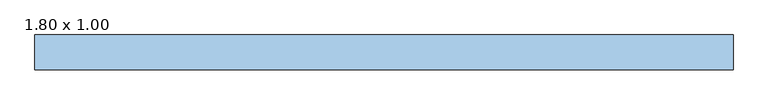
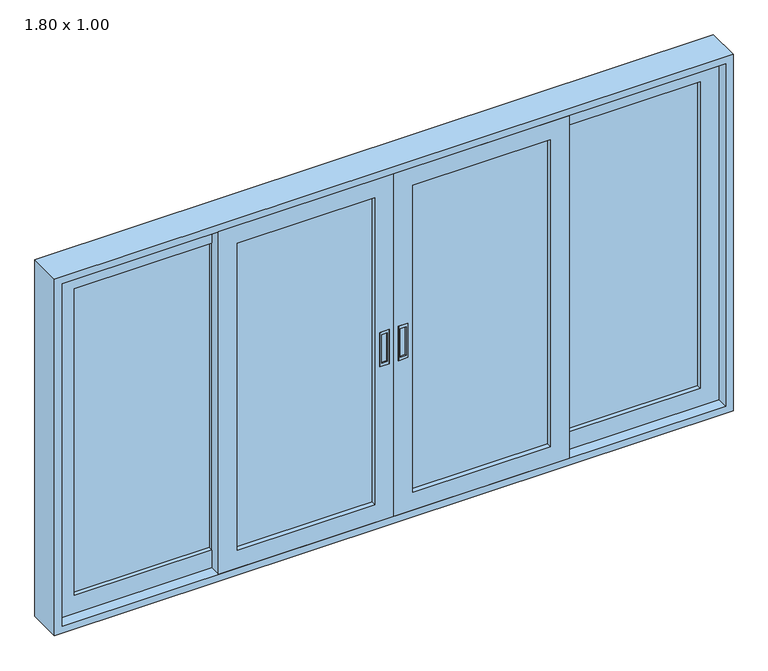
"""IFC4 building model written with IfcOpenShell, lengths in millimetres: window geometry, CC_JANELA CORRER_4 FOLHAS VIDRO : 1.80 x 1.00."""

from ifc_helpers import new_model, si_unit, frame, origin, place, context, project, spatial, polyline, outline, extrude, faceted_brep, source, transform, mapped, element, save


def window_1_80_x_1_00_ac21060c(model_context):
    return source(origin(), model_context, "Body", "SolidModel", [
        extrude(outline(polyline([(17.5, -96.0), (17.5, -95.0), (32.5, -95.0), (32.5, -96.0), (17.5, -96.0)])), frame((0.0, 0.0, 1460.0), z_axis=(0.0, 0.0, 1.0), x_axis=(1.0, 0.0, 0.0)), (0.0, 0.0, 1.0), 80.0),
        extrude(outline(polyline([(1452.0, 37.5), (1548.0, 37.5), (1548.0, 12.5), (1452.0, 12.5), (1452.0, 37.5)]), holes=[polyline([(1460.0, 32.5), (1460.0, 17.5), (1540.0, 17.5), (1540.0, 32.5), (1460.0, 32.5)])]), frame((0.0, -100.1, 0.0), z_axis=(0.0, 1.0, 0.0), x_axis=(0.0, 0.0, 1.0)), (0.0, 0.0, 1.0), 5.1),
        faceted_brep([(50.0, -100.0, 1930.0), (50.0, -100.0, 1070.0), (50.0, -70.0, 1070.0), (50.0, -70.0, 1930.0), (0.0, -70.0, 1980.0), (465.0, -70.0, 1980.0), (465.0, -70.0, 1020.0), (0.0, -70.0, 1020.0), (415.0, -70.0, 1070.0), (415.0, -70.0, 1930.0), (415.0, -100.0, 1070.0), (0.0, -100.0, 1020.0), (465.0, -100.0, 1020.0), (465.0, -100.0, 1980.0), (0.0, -100.0, 1980.0), (37.5, -100.0, 1548.0), (37.5, -100.0, 1452.0), (12.5, -100.0, 1452.0), (12.5, -100.0, 1548.0), (415.0, -100.0, 1930.0), (12.5, -95.0, 1452.0), (12.5, -95.0, 1548.0), (37.5, -95.0, 1452.0), (37.5, -95.0, 1548.0)], [[[0, 1, 2, 3]], [[4, 5, 6, 7], [2, 8, 9, 3]], [[1, 10, 8, 2]], [[11, 12, 13, 14], [15, 16, 17, 18], [0, 19, 10, 1]], [[4, 7, 11, 14]], [[7, 6, 12, 11]], [[10, 19, 9, 8]], [[6, 5, 13, 12]], [[18, 17, 20, 21]], [[20, 17, 16, 22]], [[23, 22, 16, 15]], [[21, 20, 22, 23]], [[3, 9, 19, 0]], [[14, 13, 5, 4]], [[21, 23, 15, 18]]]),
        extrude(outline(polyline([(50.0, -82.5), (415.0, -82.5), (415.0, -87.5), (50.0, -87.5), (50.0, -82.5)])), frame((0.0, 0.0, 1070.0), z_axis=(0.0, 0.0, 1.0), x_axis=(1.0, 0.0, 0.0)), (0.0, 0.0, 1.0), 860.0),
        extrude(outline(polyline([(-17.5, -96.0), (-32.5, -96.0), (-32.5, -95.0), (-17.5, -95.0), (-17.5, -96.0)])), frame((0.0, 0.0, 1460.0), z_axis=(0.0, 0.0, 1.0), x_axis=(1.0, 0.0, 0.0)), (0.0, 0.0, 1.0), 80.0),
        extrude(outline(polyline([(1452.0, -37.5), (1452.0, -12.5), (1548.0, -12.5), (1548.0, -37.5), (1452.0, -37.5)]), holes=[polyline([(1460.0, -32.5), (1540.0, -32.5), (1540.0, -17.5), (1460.0, -17.5), (1460.0, -32.5)])]), frame((0.0, -100.1, 0.0), z_axis=(0.0, 1.0, 0.0), x_axis=(0.0, 0.0, 1.0)), (0.0, 0.0, 1.0), 5.1),
        faceted_brep([(-50.0, -100.0, 1930.0), (-50.0, -70.0, 1930.0), (-50.0, -70.0, 1070.0), (-50.0, -100.0, 1070.0), (0.0, -70.0, 1980.0), (0.0, -70.0, 1020.0), (-465.0, -70.0, 1020.0), (-465.0, -70.0, 1980.0), (-415.0, -70.0, 1930.0), (-415.0, -70.0, 1070.0), (-415.0, -100.0, 1070.0), (0.0, -100.0, 1020.0), (0.0, -100.0, 1980.0), (-465.0, -100.0, 1980.0), (-465.0, -100.0, 1020.0), (-415.0, -100.0, 1930.0), (-37.5, -100.0, 1548.0), (-12.5, -100.0, 1548.0), (-12.5, -100.0, 1452.0), (-37.5, -100.0, 1452.0), (-12.5, -95.0, 1548.0), (-12.5, -95.0, 1452.0), (-37.5, -95.0, 1452.0), (-37.5, -95.0, 1548.0)], [[[0, 1, 2, 3]], [[4, 5, 6, 7], [2, 1, 8, 9]], [[3, 2, 9, 10]], [[11, 12, 13, 14], [0, 3, 10, 15], [16, 17, 18, 19]], [[4, 12, 11, 5]], [[5, 11, 14, 6]], [[10, 9, 8, 15]], [[6, 14, 13, 7]], [[17, 20, 21, 18]], [[21, 22, 19, 18]], [[23, 16, 19, 22]], [[20, 23, 22, 21]], [[1, 0, 15, 8]], [[12, 4, 7, 13]], [[20, 17, 16, 23]]]),
        extrude(outline(polyline([(-50.0, -82.5), (-50.0, -87.5), (-415.0, -87.5), (-415.0, -82.5), (-50.0, -82.5)])), frame((0.0, 0.0, 1070.0), z_axis=(0.0, 0.0, 1.0), x_axis=(1.0, 0.0, 0.0)), (0.0, 0.0, 1.0), 860.0),
        extrude(outline(polyline([(830.0, -52.5), (830.0, -57.5), (465.0, -57.5), (465.0, -52.5), (830.0, -52.5)])), frame((0.0, 0.0, 1070.0), z_axis=(0.0, 0.0, 1.0), x_axis=(1.0, 0.0, 0.0)), (0.0, 0.0, 1.0), 860.0),
        extrude(outline(polyline([(1980.0, 880.0), (1980.0, 415.0), (1020.0, 415.0), (1020.0, 880.0), (1980.0, 880.0)]), holes=[polyline([(1070.0, 830.0), (1070.0, 465.0), (1930.0, 465.0), (1930.0, 830.0), (1070.0, 830.0)])]), frame((0.0, -70.0, 0.0), z_axis=(0.0, 1.0, 0.0), x_axis=(0.0, 0.0, 1.0)), (0.0, 0.0, 1.0), 30.0),
        extrude(outline(polyline([(-465.0, -52.5), (-465.0, -57.5), (-830.0, -57.5), (-830.0, -52.5), (-465.0, -52.5)])), frame((0.0, 0.0, 1070.0), z_axis=(0.0, 0.0, 1.0), x_axis=(1.0, 0.0, 0.0)), (0.0, 0.0, 1.0), 860.0),
        extrude(outline(polyline([(1980.0, -415.0), (1980.0, -880.0), (1020.0, -880.0), (1020.0, -415.0), (1980.0, -415.0)]), holes=[polyline([(1070.0, -465.0), (1070.0, -830.0), (1930.0, -830.0), (1930.0, -465.0), (1070.0, -465.0)])]), frame((0.0, -70.0, 0.0), z_axis=(0.0, 1.0, 0.0), x_axis=(0.0, 0.0, 1.0)), (0.0, 0.0, 1.0), 30.0),
        extrude(outline(polyline([(2000.0, 900.0), (2000.0, -900.0), (1000.0, -900.0), (1000.0, 900.0), (2000.0, 900.0)]), holes=[polyline([(1980.0, 880.0), (1020.0, 880.0), (1020.0, -880.0), (1980.0, -880.0), (1980.0, 880.0)])]), frame((0.0, -100.0, 0.0), z_axis=(0.0, 1.0, 0.0), x_axis=(0.0, 0.0, 1.0)), (0.0, 0.0, 1.0), 90.0),
    ])


if __name__ == "__main__":
    model = new_model("IFC4")
    model_context = context("Model", 3, world=origin())
    ifc_project = project(units=[si_unit("LENGTHUNIT", "METRE", prefix="MILLI")], contexts=[model_context])
    site = spatial("IfcSite", under=ifc_project)
    building = spatial("IfcBuilding", under=site)
    placement = place(None, origin())
    window_1_80_x_1_00_shape = window_1_80_x_1_00_ac21060c(model_context)
    element("IfcWindow", 1, ObjectType="CC_JANELA CORRER_4 FOLHAS VIDRO : 1.80 x 1.00", at=placement, inside=building, context=model_context, shape_type="MappedRepresentation", body=[
        mapped(window_1_80_x_1_00_shape, transform((0.0, 0.0, 0.0), x_axis=(1.0, 0.0, 0.0), y_axis=(0.0, 1.0, 0.0), z_axis=(0.0, 0.0, 1.0))),
    ])
    save(model, "model.ifc")

# Revit data of these elements
# Type "CC_JANELA CORRER_4 FOLHAS VIDRO : 1.80 x 1.00"
#   Type Mark = "J4"
#   Site = "www.construir.arq.br"
#   Emprea = "Cursos Construir"
#   Criado Por = "Roberto Netto"
#   Analytic Construction = "<Nenhum>"
#   Rough Width = 1.80 m
#   Largura Moldura Folha [instance default] = 0.05 m
#   Largura Guarnição Interna [instance default] = 0.10 m
#   Largura Moldura Externa [instance default] = 0.10 m
#   Largura Folha [instance default] = 0.465 m
#   Interna [instance default] = 0.00 m
#   Externa [instance default] = 0.00 m
#   Extensão Frontal Peitoril/Pingadeira [instance default] = 0.03 m
#   Extensão Exterior Esquerda Peitoril/Pingadeira [instance default] = 0.025 m
#   Extensão Exterior Direita Peitoril/Pingadeira [instance default] = 0.025 m
#   Extensão Caixilho [instance default] = 0.03 m
#   Espessura Peitoril/Pingadeira [instance default] = 0.02 m
#   Espessura Guarnição Interna [instance default] = 0.005 m
#   Espessura Moldura Externa [instance default] = 0.01 m
#   Espessura Folha [instance default] = 0.03 m
#   Cálculo Porcentagem [instance default] = 0.00 m
#   Cálculo Abertura [instance default] = 0.00 m
#   Espessura Caixilho [instance default] = 0.02 m
#   Rough Height = 1.00 m
#   Altura Folha [instance default] = 0.96 m
#   Altura Corte [instance default] = 0.02 m
#   Height = 1.00 m
#   Width = 1.80 m
#   ----PEITORIL/PINGADEIRA--- [instance default] = 0.00 m
#   ----MOLDURA---- [instance default] = 0.00 m
#   ----GUARNIÇÃO---- [instance default] = 0.00 m
#   ----EXTENSÃO---- [instance default] = 0.00 m
#   ----CAIXILHO---- [instance default] = 0.00 m
#   -----FOLHA---- [instance default] = 0.00 m
#   Puxador [instance default] = yes
#   Peitoril/Pingadeira Vazio [instance default] = no
#   Peitoril/Pingadeira Família [instance default] = yes
#   Guarnição Interna [instance default] = yes
#   Moldura Externa Sem Peitoril [instance default] = no
#   Moldura Externa Com Peitoril [instance default] = yes
#   Moldura Externa [instance default] = yes
#   Material Vidro Folha = .VIDRO
#   Material Puxador = .ALUMÍNIO COM PINTURA ELETROSTÁTICA BRANCA
#   Material Peitoril/Pingadeira = .GRANITO BRANCO ITAÚNAS
#   Material Moldura Folha = .ALUMÍNIO COM PINTURA ELETROSTÁTICA BRANCA
#   Material Moldura Externa = .PINTURA ACRÍLICA BRANCA
#   Material Caixilho = .ALUMÍNIO COM PINTURA ELETROSTÁTICA BRANCA
#   Material Guarnição = .ALUMÍNIO COM PINTURA ELETROSTÁTICA BRANCA
#   Wall Closure = (empty or 0)
# Element 1 (IfcWindow, "CC_JANELA CORRER_4 FOLHAS VIDRO : 1.80 x 1.00")
#   Guarnição Interna = no
#   Moldura Externa Com Peitoril = no
#   Moldura Externa = no
#   Materials on its faces: ".ALUMÍNIO COM PINTURA ELETROSTÁTICA BRANCA", ".VIDRO"
# Materials
#   ".VIDRO": class "Genérico", colour RGB 198 236 255, transparency 0.95, Cost = 0
#   ".ALUMÍNIO COM PINTURA ELETROSTÁTICA BRANCA": class "CC_METAIS", colour RGB 241 241 241, transparency 0, Cost = 0
#   ".GRANITO BRANCO ITAÚNAS": class ".CC_PEDRA REVEST.", colour RGB 202 195 174, transparency 0, Description = "Granito branco Itaúnas", Uso = "Pedra", Cost = 0
#   ".PINTURA ACRÍLICA BRANCA": class ".CC_PINTURA", colour RGB 250 250 250, transparency 0, Keynote = "09910.A1", Description = "Tinta acrílica na cor branca", Cost = 0
